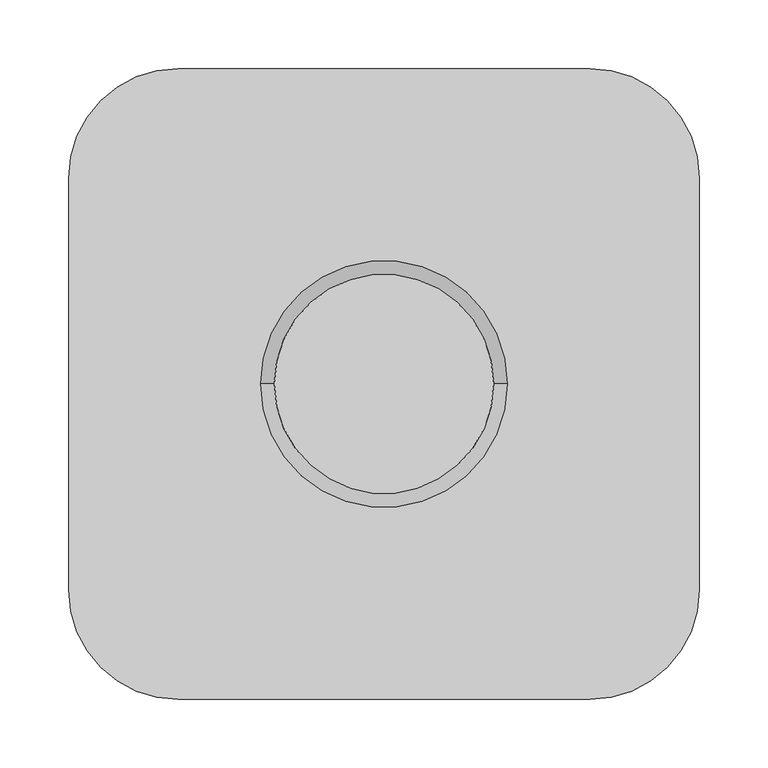
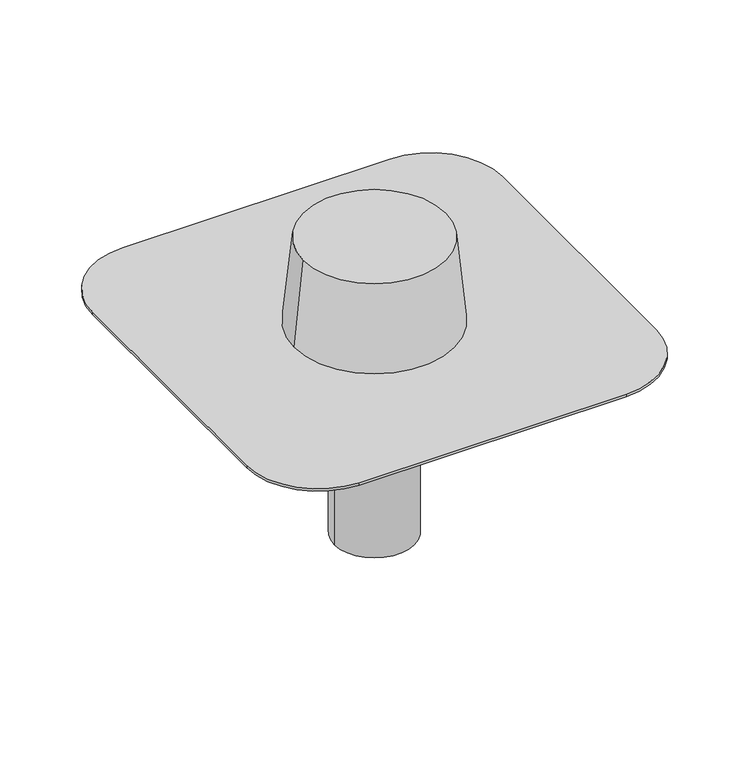
"""IFC4 building model written with IfcOpenShell, lengths in millimetres: proxy geometry, TN_ПВХ Воронка экструдированная с листоуловителем : ПВХ Воронка экструдированная ремонтная 100х240мм с листоуловителем."""

from ifc_helpers import new_model, si_unit, point, frame, frame_2d, origin, origin_2d, place, context, project, spatial, polyline, circle_curve, trimmed, segment, composite_curve, outline, extrude, source, transform, mapped, element, save
from ifc_brep_helpers import plane_surface, revolved_surface, advanced_brep


def specialty_equipment_0a6d2619(model_context):
    return source(origin(), model_context, "Body", "SolidModel", [
        extrude(outline(composite_curve([segment(trimmed(circle_curve(origin_2d(), 45.0), [point((45.0, 0.0))], [point((-45.0, 0.0))], False, "CARTESIAN"), True, "CONTINUOUS"), segment(trimmed(circle_curve(origin_2d(), 45.0), [point((-45.0, 0.0))], [point((45.0, 0.0))], False, "CARTESIAN"), True, "CONTINUOUS")], self_intersect=False)), frame((0.0, 0.0, -70.0), z_axis=(0.0, 0.0, 1.0), x_axis=(1.0, 0.0, 0.0)), (0.0, 0.0, 1.0), 20.0),
        extrude(outline(composite_curve([segment(trimmed(circle_curve(origin_2d(), 45.0), [point((-45.0, 0.0))], [point((45.0, 0.0))], False, "CARTESIAN"), True, "CONTINUOUS"), segment(trimmed(circle_curve(origin_2d(), 45.0), [point((45.0, 0.0))], [point((-45.0, 0.0))], False, "CARTESIAN"), True, "CONTINUOUS")], self_intersect=False)), frame((0.0, 0.0, -50.0), z_axis=(0.0, 0.0, 1.0), x_axis=(1.0, 0.0, 0.0)), (0.0, 0.0, 1.0), 47.0),
        extrude(outline(composite_curve([segment(trimmed(circle_curve(origin_2d(), 45.0), [point((45.0, 0.0))], [point((-45.0, 0.0))], False, "CARTESIAN"), True, "CONTINUOUS"), segment(trimmed(circle_curve(origin_2d(), 45.0), [point((-45.0, 0.0))], [point((45.0, 0.0))], False, "CARTESIAN"), True, "CONTINUOUS")], self_intersect=False)), frame((0.0, 0.0, -250.0), z_axis=(0.0, 0.0, 1.0), x_axis=(1.0, 0.0, 0.0)), (0.0, 0.0, 1.0), 180.0),
        advanced_brep(
        [(-80.0, 0.0, 100.0), (80.0, 0.0, 100.0), (-90.0, 0.0, 0.0), (90.0, 0.0, 0.0)],
        [
            (0, 1, circle_curve(frame((0.0, 0.0, 100.0), z_axis=(0.0, 0.0, 1.0), x_axis=(-1.0, 0.0, 0.0)), 80.0)),
            (1, 0, circle_curve(frame((0.0, 0.0, 100.0), z_axis=(0.0, 0.0, 1.0), x_axis=(1.0, 0.0, 0.0)), 80.0)),
            (2, 3, circle_curve(frame((0.0, 0.0, 0.0), z_axis=(0.0, 0.0, -1.0), x_axis=(1.0, 0.0, 0.0)), 90.0)),
            (3, 2, circle_curve(frame((0.0, 0.0, 0.0), z_axis=(0.0, 0.0, -1.0), x_axis=(-1.0, 0.0, 0.0)), 90.0)),
            (3, 1),
            (0, 2),
        ],
        [
            plane_surface(frame((0.0, 0.0, 100.0), z_axis=(0.0, 0.0, 1.0), x_axis=(0.0, -1.0, 0.0))),
            plane_surface(frame((0.0, 0.0, 0.0), z_axis=(0.0, 0.0, -1.0), x_axis=(0.0, -1.0, 0.0))),
            revolved_surface(polyline([(-80.0, 0.0, 100.0), (-90.0, 0.0, 0.0)]), (0.0, 0.0, 900.0), (0.0, 0.0, -1.0)),
            revolved_surface(polyline([(80.0, 0.0, 100.0), (90.0, 0.0, 0.0)]), (0.0, 0.0, 900.0), (0.0, 0.0, -1.0)),
        ],
        [
            (0, [[1, 2]]),
            (1, [[3, 4]]),
            (2, [[-4, 5, -1, 6]]),
            (3, [[-3, -6, -2, -5]]),
        ],
    ),
        extrude(outline(composite_curve([segment(trimmed(circle_curve(frame_2d((150.0, 150.0)), 80.0), [point((150.0, 230.0))], [point((230.0, 150.0))], False, "CARTESIAN"), True, "CONTINUOUS"), segment(polyline([(230.0, 150.0), (230.0, -150.0)]), True, "CONTINUOUS"), segment(trimmed(circle_curve(frame_2d((150.0, -150.0)), 80.0), [point((230.0, -150.0))], [point((150.0, -230.0))], False, "CARTESIAN"), True, "CONTINUOUS"), segment(polyline([(150.0, -230.0), (-150.0, -230.0)]), True, "CONTINUOUS"), segment(trimmed(circle_curve(frame_2d((-150.0, -150.0)), 80.0), [point((-150.0, -230.0))], [point((-230.0, -150.0))], False, "CARTESIAN"), True, "CONTINUOUS"), segment(polyline([(-230.0, -150.0), (-230.0, 150.0)]), True, "CONTINUOUS"), segment(trimmed(circle_curve(frame_2d((-150.0, 150.0)), 80.0), [point((-230.0, 150.0))], [point((-150.0, 230.0))], False, "CARTESIAN"), True, "CONTINUOUS"), segment(polyline([(-150.0, 230.0), (150.0, 230.0)]), True, "CONTINUOUS")], self_intersect=False)), frame((0.0, 0.0, -3.0), z_axis=(0.0, 0.0, 1.0), x_axis=(1.0, 0.0, 0.0)), (0.0, 0.0, 1.0), 3.0),
    ])


if __name__ == "__main__":
    model = new_model("IFC4")
    model_context = context("Model", 3, world=origin())
    ifc_project = project(units=[si_unit("LENGTHUNIT", "METRE", prefix="MILLI")], contexts=[model_context])
    site = spatial("IfcSite", under=ifc_project)
    building = spatial("IfcBuilding", under=site)
    placement = place(None, origin())
    specialty_equipment_shape = specialty_equipment_0a6d2619(model_context)
    element("IfcBuildingElementProxy", 1, Name="TN_ПВХ Воронка экструдированная с листоуловителем : ПВХ Воронка экструдированная ремонтная 100х240мм с листоуловителем", ObjectType="TN_ПВХ Воронка экструдированная с листоуловителем : ПВХ Воронка экструдированная ремонтная 100х240мм с листоуловителем", at=placement, inside=building, context=model_context, shape_type="MappedRepresentation", body=[
        mapped(specialty_equipment_shape, transform((0.0, 0.0, 0.0), x_axis=(1.0, 0.0, 0.0), y_axis=(0.0, 1.0, 0.0), z_axis=(0.0, 0.0, 1.0))),
    ])
    save(model, "model.ifc")

# Revit data of these elements
# Type "TN_ПВХ Воронка экструдированная с листоуловителем : ПВХ Воронка экструдированная ремонтная 100х240мм с листоуловителем"
#   ADSK_Группирование = "Комплектующие и воронки"
#   Description = "Экструдированная ПВХ воронка 100х240мм ТехноНИКОЛЬ – кровельная воронка с листвоуловителем применяется совместно с ПВХ мембранами LOGICROOF и ECOPLAST. Приваривается к мембране гомогенно при помощи горячего воздуха. Масса 510 г."
#   Manufacturer = "ТехноНИКОЛЬ"
#   URL = "http://nav.tn.ru/upload/iblock/9b8/Tekhlist-7.50_PVKH-voronka-ekstrudirovannaya_rus.pdf"
#   ADSK_Примечание = ""
#   ADSK_Обозначение = "ТехноНИКОЛЬ"
#   ADSK_Наименование = "ПВХ Воронка экструдированная ремонтная 100х240мм с листоуловителем"
#   ADSK_Марка = ""
#   ADSK_Код изделия = "361585"
#   ADSK_Завод-изготовитель = "ТехноНИКОЛЬ"
#   ADSK_Единица измерения = "шт."
#   ADSK_Группирование = "Комплектующие и воронки"
#   ADSK_URL страницы изделия = "https://shop.tn.ru/pvh-voronka-jekstrudirovannaja-100h240-mm"
#   ADSK_URL документации изделия = "https://nav.tn.ru/upload/iblock/8ec/Tekhlist-7.50_PVKH-voronka-ekstrudirovannaya_rus.pdf"
#   Радиус воронки низ = 45 mm
#   Радиус воронки верх = 45 mm
#   Default Elevation = 1219.2 mm
#   Длина расчетная [instance default] = 250 mm
#   Длина отвода [instance default] = 250 mm
#   Диаметр защитной решетки низ = 180 mm
#   Диаметр защитной решетки верх = 160 mm
#   Диаметр воронки низ = 90 mm
#   Диаметр воронки верх = 90 mm
#   ADSK_Масса = 0.73
#   ADSK_Количество = 1
#   Материал B = TN_ПВХ_Черный
#   Материал A = TN_ПВХ_Серый
# Element 1 (IfcBuildingElementProxy, "TN_ПВХ Воронка экструдированная с листоуловителем : ПВХ Воронка экструдированная ремонтная 100х240мм с листоуловителем")
#   Materials on its faces: "TN_ПВХ_Серый", "TN_ПВХ_Черный"
# Materials
#   "TN_ПВХ_Черный": class "Типовые", colour RGB 48 48 48, transparency 0, Cost = 0
#   "TN_ПВХ_Серый": class "Типовые", colour RGB 192 192 192, transparency 0, Cost = 0
